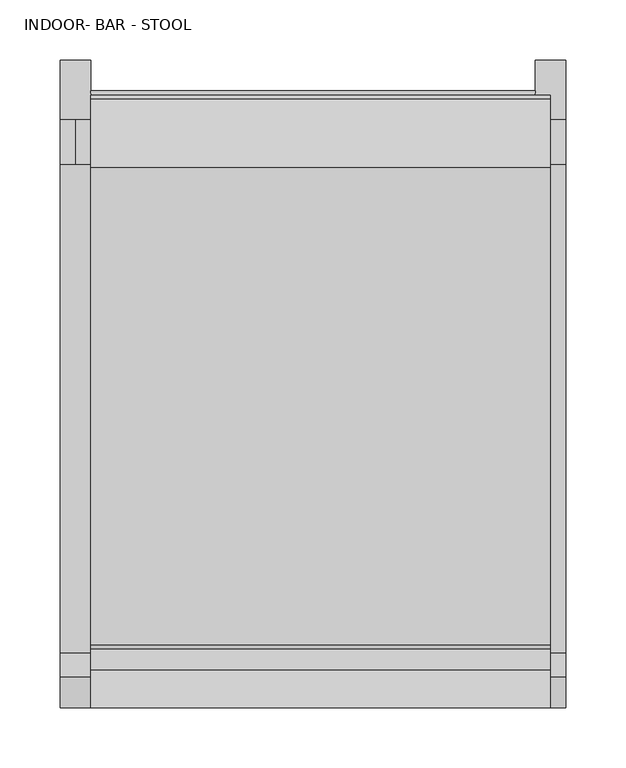
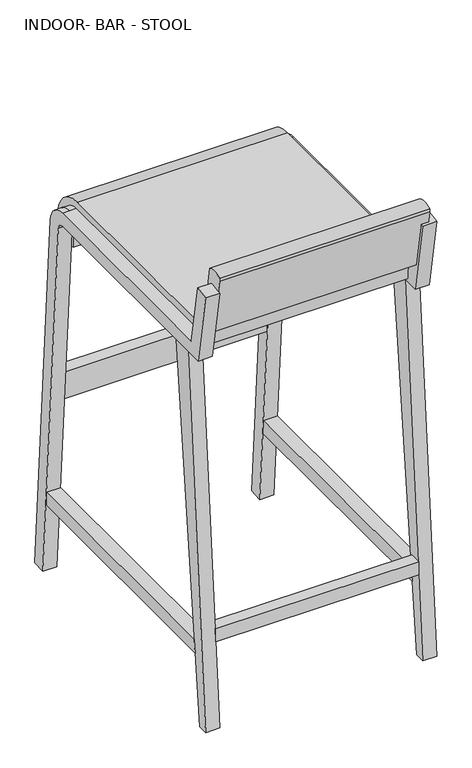
"""IFC4 building model written with IfcOpenShell, lengths in millimetres: furniture geometry, Bar_Stool_6722[1]1 : INDOOR- BAR - STOOL."""

from ifc_helpers import new_model, si_unit, point, frame, frame_2d, origin, place, context, project, spatial, polyline, circle_curve, trimmed, segment, composite_curve, outline, extrude, source, transform, mapped, element, save
from ifc_brep_helpers import plane_surface, cylinder_surface, revolved_surface, advanced_brep


def indoor_bar_stool_48a66dd3(model_context):
    return source(origin(), model_context, "Body", "SolidModel", [
        advanced_brep(
        [(419.1, 25.0141169, 838.4759165), (393.7, 25.0141169, 838.4759165), (393.7, 0.0, 834.0652528), (419.1, 0.0, 834.0652528), (419.1, 45.2169423, 723.9), (393.7, 45.2169423, 723.9), (393.7, 450.0350637, 723.9), (393.7, 488.0397183, 688.4937383), (393.7, 536.7759384, 0.8979128), (393.7, 511.439502, -0.8979128), (393.7, 462.7032819, 686.6979128), (393.7, 450.0350637, 698.5), (393.7, 23.9038117, 698.5), (419.1, 23.9038117, 698.5), (419.1, 450.0350637, 698.5), (419.1, 462.7032819, 686.6979128), (419.1, 511.439502, -0.8979128), (419.1, 536.7759384, 0.8979128), (419.1, 488.0397183, 688.4937383), (419.1, 450.0350637, 723.9), (406.4, 450.0350637, 723.9), (406.4, 488.0397183, 688.4937383)],
        [
            (0, 1),
            (1, 2),
            (2, 3),
            (3, 0),
            (0, 4),
            (4, 5),
            (5, 1),
            (5, 6),
            (6, 7, circle_curve(frame((393.7, 450.0350637, 685.8), z_axis=(-1.0, 0.0, 0.0), x_axis=(0.0, 0.0, 1.0)), 38.1)),
            (7, 8),
            (8, 9),
            (9, 10),
            (10, 11, circle_curve(frame((393.7, 450.0350637, 685.8), z_axis=(1.0, 0.0, 0.0), x_axis=(0.0, 0.0, 1.0)), 12.7)),
            (11, 12),
            (12, 2),
            (12, 13),
            (13, 3),
            (13, 14),
            (14, 15, circle_curve(frame((419.1, 450.0350637, 685.8), z_axis=(-1.0, 0.0, 0.0), x_axis=(0.0, 0.0, 1.0)), 12.7)),
            (15, 16),
            (16, 17),
            (17, 18),
            (18, 19, circle_curve(frame((419.1, 450.0350637, 685.8), z_axis=(1.0, 0.0, 0.0), x_axis=(0.0, 0.0, 1.0)), 38.1)),
            (19, 4),
            (19, 20),
            (20, 6),
            (11, 14),
            (21, 20, circle_curve(frame((406.4, 450.0350637, 685.8), z_axis=(1.0, 0.0, 0.0), x_axis=(0.0, 0.0, 1.0)), 38.1)),
            (18, 21),
            (21, 7),
            (10, 15),
            (17, 8),
            (9, 16),
        ],
        [
            plane_surface(frame((406.4, 12.5070585, 836.2705846), z_axis=(0.0, -0.17364817766692853, 0.9848077530122085), x_axis=(1.0, 0.0, 0.0))),
            plane_surface(frame((406.4, 25.0141169, 838.4759165), z_axis=(0.0, 0.9848077530122085, 0.17364817766692814), x_axis=(0.0, 0.17364817766692814, -0.9848077530122085))),
            plane_surface(frame((393.7, 25.0141169, 838.4759165), z_axis=(-1.0, 0.0, 0.0), x_axis=(0.0, 0.17364817766692808, -0.9848077530122085))),
            plane_surface(frame((393.7, 0.0, 834.0652528), z_axis=(0.0, -0.9848077530122085, -0.17364817766692817), x_axis=(0.0, 0.17364817766692817, -0.9848077530122085))),
            plane_surface(frame((419.1, 0.0, 834.0652528), z_axis=(1.0000000000000002, 0.0, 0.0), x_axis=(0.0, 0.1736481776669284, -0.9848077530122085))),
            plane_surface(frame((406.4, 45.2169423, 723.9), z_axis=(0.0, 0.0, 1.0), x_axis=(0.0, 1.0, 0.0))),
            plane_surface(frame((393.7, 23.9038117, 698.5), z_axis=(0.0, 0.0, -1.0), x_axis=(0.0, 1.0, 0.0))),
            cylinder_surface(frame((406.4, 450.0350637, 685.8), z_axis=(-1.0, 0.0, 0.0), x_axis=(0.0, 0.0, 1.0)), 38.1),
            revolved_surface(polyline([(393.7, 450.0350637, 698.5), (419.1, 450.0350637, 698.5)]), (406.4, 450.0350637, 685.8), (-1.0, 0.0, 0.0)),
            plane_surface(frame((406.4, 488.0397183, 688.4937383), z_axis=(0.0, 0.9974974969901172, 0.07070179275273744), x_axis=(0.0, 0.07070179275273744, -0.9974974969901172))),
            plane_surface(frame((393.7, 462.7032819, 686.6979128), z_axis=(0.0, -0.9974974969901172, -0.07070179275273743), x_axis=(0.0, 0.07070179275273743, -0.9974974969901172))),
            plane_surface(frame((406.4, 524.1077202, 0.0), z_axis=(0.0, 0.07070179275273399, -0.9974974969901175), x_axis=(1.0, 0.0, 0.0))),
        ],
        [
            (0, [[1, 2, 3, 4]]),
            (1, [[5, 6, 7, -1]]),
            (2, [[-2, -7, 8, 9, 10, 11, 12, 13, 14, 15]]),
            (3, [[-3, -15, 16, 17]]),
            (4, [[-4, -17, 18, 19, 20, 21, 22, 23, 24, -5]]),
            (5, [[-6, -24, 25, 26, -8]]),
            (6, [[-16, -14, 27, -18]]),
            (7, [[28, -25, -23, 29]]),
            (7, [[-9, -26, -28, 30]]),
            (8, [[-19, -27, -13, 31]]),
            (9, [[-10, -30, -29, -22, 32]]),
            (10, [[-20, -31, -12, 33]]),
            (11, [[-32, -21, -33, -11]]),
        ],
    ),
        extrude(outline(composite_curve([segment(polyline([(48.4096386, 756.5644068), (44.0710693, 752.2258375), (19.1416957, 748.2774126), (0.0, 856.8353632), (0.0, 863.1853632)]), True, "CONTINUOUS"), segment(trimmed(circle_curve(frame_2d((15.7612691, 828.3540875)), 38.2313401), [point((0.0, 863.1853632))], [point((31.5225381, 863.1853632))], False, "CARTESIAN"), True, "CONTINUOUS"), segment(polyline([(31.5225381, 863.1853632), (48.4096386, 756.5644068)]), True, "CONTINUOUS")], self_intersect=False)), frame((25.4, 0.0, 0.0), z_axis=(1.0, 0.0, 0.0), x_axis=(0.0, 1.0, 0.0)), (0.0, 0.0, 1.0), 381.0),
        extrude(outline(composite_curve([segment(polyline([(51.6744261, 737.5144068), (447.8968201, 737.5144068)]), True, "CONTINUOUS"), segment(trimmed(circle_curve(frame_2d((447.8968201, 676.6245275)), 60.8898793), [point((447.8968201, 737.5144068))], [point((505.1145904, 697.4500928))], False, "CARTESIAN"), True, "CONTINUOUS"), segment(trimmed(circle_curve(frame_2d((460.5585493, 681.23302)), 47.4155486), [point((505.1145904, 697.4500928))], [point((484.2663236, 640.1699505))], False, "CARTESIAN"), True, "CONTINUOUS"), segment(polyline([(484.2663236, 640.1699505), (460.5585493, 643.13302), (460.5585493, 681.23302), (452.817441, 704.85), (46.417441, 704.85), (43.9498561, 733.0546243), (51.6744261, 737.5144068)]), True, "CONTINUOUS")], self_intersect=False)), frame((25.4, 0.0, 0.0), z_axis=(1.0, 0.0, 0.0), x_axis=(0.0, 1.0, 0.0)), (0.0, 0.0, 1.0), 381.0),
        extrude(outline(polyline([(393.7, 11.6871233), (25.4, 11.6871233), (25.4, 33.1441574), (393.7, 33.1441574), (393.7, 11.6871233)])), frame((0.0, 0.0, 157.9619127), z_axis=(0.0, 0.0, 1.0), x_axis=(1.0, 0.0, 0.0)), (0.0, 0.0, 1.0), 25.4),
        extrude(outline(polyline([(393.7, 488.2695397), (25.4, 488.2695397), (25.4, 511.439502), (393.7, 511.439502), (393.7, 488.2695397)])), frame((0.0, 0.0, 335.7619127), z_axis=(0.0, 0.0, 1.0), x_axis=(1.0, 0.0, 0.0)), (0.0, 0.0, 1.0), 50.8),
        extrude(outline(polyline([(500.1796497, 157.9619127), (500.1796497, 132.5619127), (32.9828185, 132.5619127), (35.652466, 157.9619127), (500.1796497, 157.9619127)])), frame((393.7, 0.0, 0.0), z_axis=(1.0, 0.0, 0.0), x_axis=(0.0, 1.0, 0.0)), (0.0, 0.0, 1.0), 25.4),
        extrude(outline(polyline([(500.1796497, 157.9619127), (500.1796497, 132.5619127), (32.9828185, 132.5619127), (35.652466, 157.9619127), (500.1796497, 157.9619127)])), frame((0.0, 0.0, 0.0), z_axis=(1.0, 0.0, 0.0), x_axis=(0.0, 1.0, 0.0)), (0.0, 0.0, 1.0), 25.4),
        extrude(outline(polyline([(0.0, 0.0), (55.3031462, 698.5), (92.4653083, 698.5), (19.05, 0.0), (0.0, 0.0)])), frame((393.7, 0.0, 0.0), z_axis=(1.0, 0.0, 0.0), x_axis=(0.0, 1.0, 0.0)), (0.0, 0.0, 1.0), 25.4),
        advanced_brep(
        [(25.4, 25.0141169, 838.4759165), (0.0, 25.0141169, 838.4759165), (0.0, 0.0, 834.0652528), (25.4, 0.0, 834.0652528), (25.4, 45.2169423, 723.9), (0.0, 45.2169423, 723.9), (0.0, 450.0350637, 723.9), (0.0, 488.0397183, 688.4937383), (0.0, 536.7759384, 0.8979128), (0.0, 511.439502, -0.8979128), (0.0, 462.7032819, 686.6979128), (0.0, 450.0350637, 698.5), (0.0, 23.9038117, 698.5), (25.4, 23.9038117, 698.5), (25.4, 450.0350637, 698.5), (25.4, 462.7032819, 686.6979128), (25.4, 511.439502, -0.8979128), (25.4, 536.7759384, 0.8979128), (25.4, 488.0397183, 688.4937383), (25.4, 450.0350637, 723.9), (12.7, 450.0350637, 723.9), (12.7, 488.0397183, 688.4937383)],
        [
            (0, 1),
            (1, 2),
            (2, 3),
            (3, 0),
            (0, 4),
            (4, 5),
            (5, 1),
            (5, 6),
            (6, 7, circle_curve(frame((0.0, 450.0350637, 685.8), z_axis=(-1.0, 0.0, 0.0), x_axis=(0.0, 0.0, 1.0)), 38.1)),
            (7, 8),
            (8, 9),
            (9, 10),
            (10, 11, circle_curve(frame((0.0, 450.0350637, 685.8), z_axis=(1.0, 0.0, 0.0), x_axis=(0.0, 0.0, 1.0)), 12.7)),
            (11, 12),
            (12, 2),
            (12, 13),
            (13, 3),
            (13, 14),
            (14, 15, circle_curve(frame((25.4, 450.0350637, 685.8), z_axis=(-1.0, 0.0, 0.0), x_axis=(0.0, 0.0, 1.0)), 12.7)),
            (15, 16),
            (16, 17),
            (17, 18),
            (18, 19, circle_curve(frame((25.4, 450.0350637, 685.8), z_axis=(1.0, 0.0, 0.0), x_axis=(0.0, 0.0, 1.0)), 38.1)),
            (19, 4),
            (19, 20),
            (20, 6),
            (11, 14),
            (21, 20, circle_curve(frame((12.7, 450.0350637, 685.8), z_axis=(1.0, 0.0, 0.0), x_axis=(0.0, 0.0, 1.0)), 38.1)),
            (18, 21),
            (21, 7),
            (10, 15),
            (17, 8),
            (9, 16),
        ],
        [
            plane_surface(frame((12.7, 12.5070585, 836.2705846), z_axis=(0.0, -0.17364817766692853, 0.9848077530122085), x_axis=(1.0, 0.0, 0.0))),
            plane_surface(frame((12.7, 25.0141169, 838.4759165), z_axis=(0.0, 0.9848077530122085, 0.173648177666928), x_axis=(0.0, 0.173648177666928, -0.9848077530122085))),
            plane_surface(frame((0.0, 25.0141169, 838.4759165), z_axis=(-1.0, 0.0, 0.0), x_axis=(0.0, 0.17364817766692875, -0.9848077530122084))),
            plane_surface(frame((0.0, 0.0, 834.0652528), z_axis=(0.0, -0.9848077530122084, -0.17364817766692883), x_axis=(0.0, 0.17364817766692883, -0.9848077530122084))),
            plane_surface(frame((25.4, 0.0, 834.0652528), z_axis=(1.0000000000000002, 0.0, 0.0), x_axis=(0.0, 0.1736481776669284, -0.9848077530122085))),
            plane_surface(frame((12.7, 45.2169423, 723.9), z_axis=(0.0, 0.0, 1.0), x_axis=(0.0, 1.0, 0.0))),
            plane_surface(frame((0.0, 23.9038117, 698.5), z_axis=(0.0, 0.0, -1.0), x_axis=(0.0, 1.0, 0.0))),
            cylinder_surface(frame((12.7, 450.0350637, 685.8), z_axis=(-1.0, 0.0, 0.0), x_axis=(0.0, 0.0, 1.0)), 38.1),
            revolved_surface(polyline([(0.0, 450.0350637, 698.5), (25.4, 450.0350637, 698.5)]), (12.7, 450.0350637, 685.8), (-1.0, 0.0, 0.0)),
            plane_surface(frame((12.7, 488.0397183, 688.4937383), z_axis=(0.0, 0.9974974969901172, 0.07070179275273744), x_axis=(0.0, 0.07070179275273744, -0.9974974969901172))),
            plane_surface(frame((0.0, 462.7032819, 686.6979128), z_axis=(0.0, -0.9974974969901172, -0.07070179275273743), x_axis=(0.0, 0.07070179275273743, -0.9974974969901172))),
            plane_surface(frame((12.7, 524.1077202, 0.0), z_axis=(0.0, 0.07070179275273399, -0.9974974969901175), x_axis=(1.0, 0.0, 0.0))),
        ],
        [
            (0, [[1, 2, 3, 4]]),
            (1, [[5, 6, 7, -1]]),
            (2, [[-2, -7, 8, 9, 10, 11, 12, 13, 14, 15]]),
            (3, [[-3, -15, 16, 17]]),
            (4, [[-4, -17, 18, 19, 20, 21, 22, 23, 24, -5]]),
            (5, [[-6, -24, 25, 26, -8]]),
            (6, [[-16, -14, 27, -18]]),
            (7, [[28, -25, -23, 29]]),
            (7, [[-9, -26, -28, 30]]),
            (8, [[-19, -27, -13, 31]]),
            (9, [[-10, -30, -29, -22, 32]]),
            (10, [[-20, -31, -12, 33]]),
            (11, [[-32, -21, -33, -11]]),
        ],
    ),
        extrude(outline(polyline([(0.0, 0.0), (55.3031462, 698.5), (92.4653083, 698.5), (19.05, 0.0), (0.0, 0.0)])), frame((0.0, 0.0, 0.0), z_axis=(1.0, 0.0, 0.0), x_axis=(0.0, 1.0, 0.0)), (0.0, 0.0, 1.0), 25.4),
    ])


if __name__ == "__main__":
    model = new_model("IFC4")
    model_context = context("Model", 3, world=origin())
    ifc_project = project(units=[si_unit("LENGTHUNIT", "METRE", prefix="MILLI")], contexts=[model_context])
    site = spatial("IfcSite", under=ifc_project)
    building = spatial("IfcBuilding", under=site)
    placement = place(None, origin())
    indoor_bar_stool_shape = indoor_bar_stool_48a66dd3(model_context)
    element("IfcFurniture", 1, ObjectType="Bar_Stool_6722[1]1 : INDOOR- BAR - STOOL", at=placement, inside=building, context=model_context, shape_type="MappedRepresentation", body=[
        mapped(indoor_bar_stool_shape, transform((0.0, 0.0, 0.0), x_axis=(1.0, 0.0, 0.0), y_axis=(0.0, 1.0, 0.0), z_axis=(0.0, 0.0, 1.0))),
    ])
    save(model, "model.ifc")

# Revit data of these elements
# Type "Bar_Stool_6722[1]1 : INDOOR- BAR - STOOL"
#   Type Mark = "TYPE - INDOOR - BAR - STOOL"
#   Seating Count = 1
#   Seat = fab
#   Chair Legs = MET
# Element 1 (IfcFurniture, "Bar_Stool_6722[1]1 : INDOOR- BAR - STOOL")
#   Materials on its faces: "MET", "fab"
# Materials
#   "fab": class "Leather", colour RGB 255 255 255, transparency 0, Cost = 0
#   "MET": class "Metal", colour RGB 189 187 185, transparency 0
